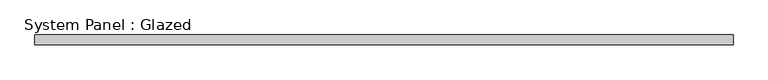
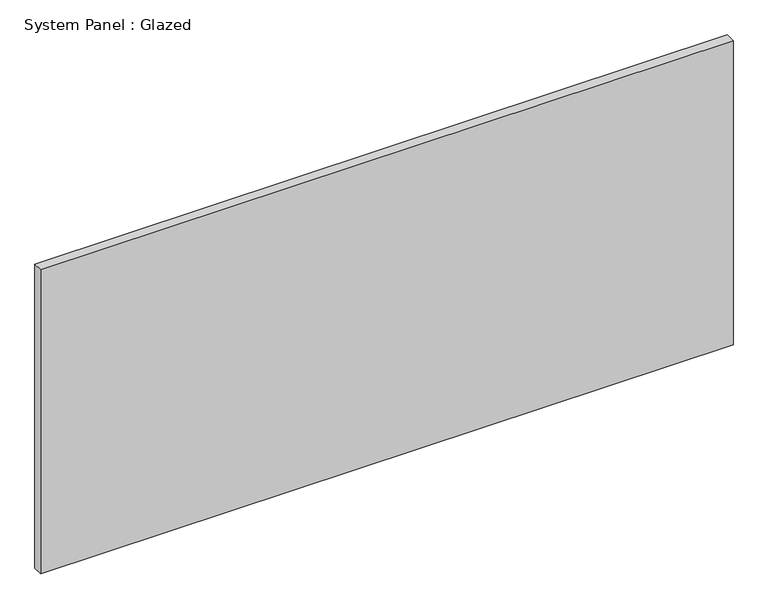
"""IFC4 building model written with IfcOpenShell, lengths in millimetres: plate geometry, System Panel : Glazed."""

from ifc_helpers import new_model, si_unit, origin, origin_with_axes, place, context, project, spatial, polyline, outline, extrude, source, transform, mapped, element, save


def system_panel_glazed_f11ab94e(model_context):
    return source(origin(), model_context, "Body", "SweptSolid", [
        extrude(outline(polyline([(882.65, -44.45), (-882.65, -44.45), (-882.65, -19.05), (882.65, -19.05), (882.65, -44.45)])), origin_with_axes(), (0.0, 0.0, 1.0), 819.15),
    ])


if __name__ == "__main__":
    model = new_model("IFC4")
    model_context = context("Model", 3, world=origin())
    ifc_project = project(units=[si_unit("LENGTHUNIT", "METRE", prefix="MILLI")], contexts=[model_context])
    site = spatial("IfcSite", under=ifc_project)
    building = spatial("IfcBuilding", under=site)
    placement = place(None, origin())
    system_panel_glazed_shape = system_panel_glazed_f11ab94e(model_context)
    element("IfcPlate", 1, ObjectType="System Panel : Glazed", at=placement, inside=building, context=model_context, shape_type="MappedRepresentation", body=[
        mapped(system_panel_glazed_shape, transform((0.0, 0.0, 0.0), x_axis=(1.0, 0.0, 0.0), y_axis=(0.0, 1.0, 0.0), z_axis=(0.0, 0.0, 1.0))),
    ])
    save(model, "model.ifc")

# Revit data of these elements
# Type "System Panel : Glazed"
#   Construction Type Id = "GSP4R"
#   Analytic Construction = "1/8 in Pilkington single glazing"
#   Visual Light Transmittance = 0.9
#   Solar Heat Gain Coefficient = 0.86
#   Heat Transfer Coefficient (U) = 1.18115 BTU/(h·ft²·°F)
#   Define Thermal Properties by = 1
# Element 1 (IfcPlate, "System Panel : Glazed")
#   Materials on its faces: "Glass"
# Materials
#   "Glass": class "Glass", colour RGB 0 128 192, transparency 0.75, Description = "Soda Lime Glass", Cost = 0
